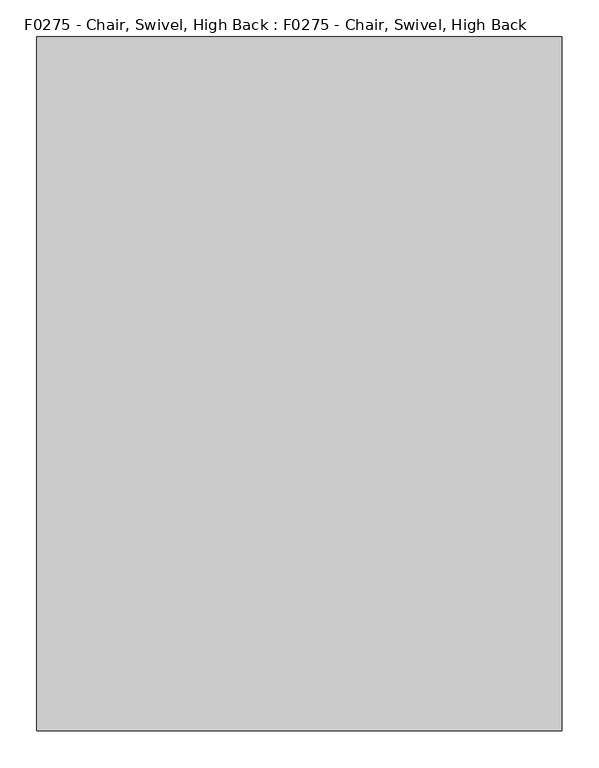
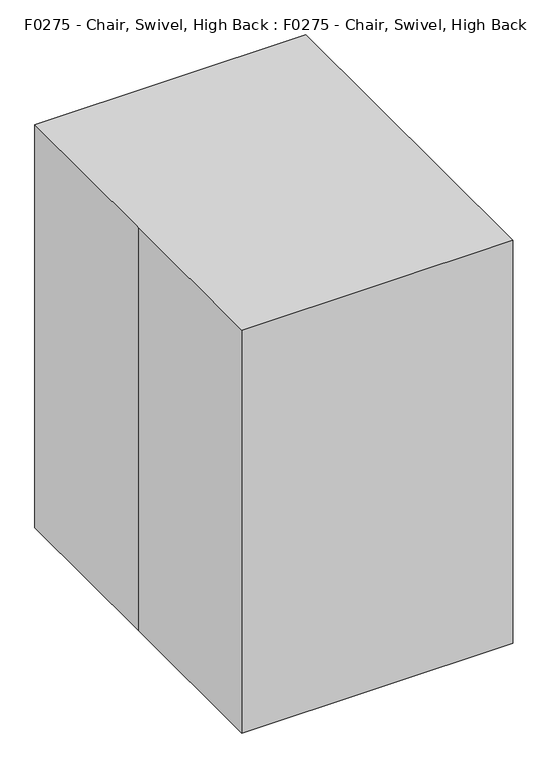
"""IFC4 building model written with IfcOpenShell, lengths in millimetres: proxy geometry, F0275 - Chair, Swivel, High Back : F0275 - Chair, Swivel, High Back."""

import ifcopenshell
import ifcopenshell.guid

model = None  # the IFC model being written
_history = None  # IfcOwnerHistory: only IFC2X3 demands one
_inside = {}  # id of a spatial element -> (the spatial element, [elements in it])
_under = {}  # id of a project, library or spatial element -> (it, [spatial elements below it])
_declared = {}  # id of a project -> (the project, [libraries it declares])
_typed = {}  # id of a type object -> (the type object, [elements of that type])
_made_of = {}  # id of a material, layer set ... -> (it, [elements and type objects made of it])


def new_model(schema):
    """Start an empty IFC model of exactly this schema.

    Asked for "IFC4X3", IfcOpenShell would pick the latest addendum, in which some entities
    have other attributes; the version numbers below select the first issue.
    IFC2X3 requires an IfcOwnerHistory on every rooted entity: one is made here for all.
    """
    global model, _history
    if schema == "IFC4X3":
        model = ifcopenshell.file(schema_version=(4, 3, 0, 0))
    else:
        model = ifcopenshell.file(schema=schema)
    _inside.clear()
    _under.clear()
    _declared.clear()
    _typed.clear()
    _made_of.clear()
    _history = None
    if model.schema == "IFC2X3":
        org = make("IfcOrganization", Name="unknown")
        user = make(
            "IfcPersonAndOrganization",
            ThePerson=make("IfcPerson", FamilyName="unknown"),
            TheOrganization=org,
        )
        app = make(
            "IfcApplication",
            ApplicationDeveloper=org,
            Version="unknown",
            ApplicationFullName="unknown",
            ApplicationIdentifier="unknown",
        )
        _history = make(
            "IfcOwnerHistory",
            OwningUser=user,
            OwningApplication=app,
            ChangeAction="ADDED",
            CreationDate=0,
        )
    return model


def make(cls, **values):
    """One entity of the class cls with the attributes given. An attribute that is None is left unset."""
    return model.create_entity(
        cls, **{name: value for name, value in values.items() if value is not None}
    )


def rooted(cls, **values):
    """An entity with a GlobalId (a new one), such as an element, a storey or a relation."""
    return make(cls, GlobalId=ifcopenshell.guid.new(), OwnerHistory=_history, **values)


def si_unit(unit_type, name, prefix=None):
    """IfcSIUnit, for example si_unit("LENGTHUNIT", "METRE", prefix="MILLI")."""
    return make("IfcSIUnit", UnitType=unit_type, Prefix=prefix, Name=name)


def assignment(units):
    """IfcUnitAssignment: the units of a project."""
    return None if units is None else make("IfcUnitAssignment", Units=units)


def point(xyz):
    """IfcCartesianPoint."""
    return None if xyz is None else make("IfcCartesianPoint", Coordinates=xyz)


def direction(xyz):
    """IfcDirection."""
    return None if xyz is None else make("IfcDirection", DirectionRatios=xyz)


def frame(location, z_axis=None, x_axis=None):
    """IfcAxis2Placement3D, a coordinate frame: its origin and axes. An axis left out is left unset."""
    return make(
        "IfcAxis2Placement3D",
        Location=point(location),
        Axis=direction(z_axis),
        RefDirection=direction(x_axis),
    )


def frame_2d(location, x_axis=None):
    """IfcAxis2Placement2D, a coordinate frame in the plane: its origin and x axis."""
    return make(
        "IfcAxis2Placement2D", Location=point(location), RefDirection=direction(x_axis)
    )


def origin():
    """The frame at (0, 0, 0) with its axes left unset."""
    return frame((0.0, 0.0, 0.0))


def origin_with_axes():
    """The frame at (0, 0, 0) with the z axis (0, 0, 1) and the x axis (1, 0, 0) written out."""
    return frame((0.0, 0.0, 0.0), z_axis=(0.0, 0.0, 1.0), x_axis=(1.0, 0.0, 0.0))


def place(relative_to, where):
    """IfcLocalPlacement: puts the frame where relative to a parent placement (None: the world)."""
    return make(
        "IfcLocalPlacement", PlacementRelTo=relative_to, RelativePlacement=where
    )


def context(
    kind, dimensions, precision=None, world=None, true_north=None, identifier=None
):
    """IfcGeometricRepresentationContext, for example the 3D "Model" context."""
    return make(
        "IfcGeometricRepresentationContext",
        ContextIdentifier=identifier,
        ContextType=kind,
        CoordinateSpaceDimension=dimensions,
        Precision=precision,
        WorldCoordinateSystem=world,
        TrueNorth=true_north,
    )


def project(units=None, contexts=None):
    """IfcProject with its units and contexts."""
    return rooted(
        "IfcProject",
        Name="project",
        RepresentationContexts=contexts,
        UnitsInContext=assignment(units),
    )


def spatial(cls, under=None, at=None, **own):
    """A site, building, storey or space (cls), placed at a placement, below another one or the project."""
    s = rooted(cls, ObjectPlacement=at, **own)
    if under is not None:
        _under.setdefault(under.id(), (under, []))[1].append(s)
    return s


def polyline(points):
    """IfcPolyline through the points."""
    return make("IfcPolyline", Points=[point(p) for p in points])


def circle_curve(where, radius):
    """IfcCircle in the frame where."""
    return make("IfcCircle", Position=where, Radius=radius)


def ellipse_curve(where, semi_axis1, semi_axis2):
    """IfcEllipse in the frame where."""
    return make(
        "IfcEllipse", Position=where, SemiAxis1=semi_axis1, SemiAxis2=semi_axis2
    )


def trimmed(basis, trim1, trim2, sense, master):
    """IfcTrimmedCurve: the piece of a basis curve between two trims."""
    return make(
        "IfcTrimmedCurve",
        BasisCurve=basis,
        Trim1=trim1,
        Trim2=trim2,
        SenseAgreement=sense,
        MasterRepresentation=master,
    )


def segment(curve, same_sense, transition):
    """IfcCompositeCurveSegment."""
    return make(
        "IfcCompositeCurveSegment",
        Transition=transition,
        SameSense=same_sense,
        ParentCurve=curve,
    )


def composite_curve(segments, self_intersect=None):
    """IfcCompositeCurve: segments joined end to end."""
    return make("IfcCompositeCurve", Segments=segments, SelfIntersect=self_intersect)


def outline(outer, holes=None, kind="AREA"):
    """IfcArbitraryClosedProfileDef: a profile drawn as a closed curve; with holes, ...WithVoids."""
    if holes is None:
        return make("IfcArbitraryClosedProfileDef", ProfileType=kind, OuterCurve=outer)
    return make(
        "IfcArbitraryProfileDefWithVoids",
        ProfileType=kind,
        OuterCurve=outer,
        InnerCurves=holes,
    )


def extrude(swept, where, along, depth):
    """IfcExtrudedAreaSolid: the profile swept, set in the frame where, extruded along a direction by depth."""
    return make(
        "IfcExtrudedAreaSolid",
        SweptArea=swept,
        Position=where,
        ExtrudedDirection=direction(along),
        Depth=depth,
    )


def shape(context_of_items, identifier, shape_type, items):
    """IfcShapeRepresentation: the items that make up one representation, for example the "Body"."""
    return make(
        "IfcShapeRepresentation",
        ContextOfItems=context_of_items,
        RepresentationIdentifier=identifier,
        RepresentationType=shape_type,
        Items=items,
    )


def source(mapping_origin, context_of_items, identifier, shape_type, items):
    """IfcRepresentationMap: a shape defined once, which mapped items show again and again."""
    return make(
        "IfcRepresentationMap",
        MappingOrigin=mapping_origin,
        MappedRepresentation=shape(context_of_items, identifier, shape_type, items),
    )


def transform(
    local_origin,
    x_axis=None,
    y_axis=None,
    z_axis=None,
    scale=None,
    scale2=None,
    scale3=None,
    uniform=True,
):
    """IfcCartesianTransformationOperator3D, or its non-uniform kind. x_axis, y_axis, z_axis: its Axis1, 2, 3."""
    if uniform:
        return make(
            "IfcCartesianTransformationOperator3D",
            Axis1=direction(x_axis),
            Axis2=direction(y_axis),
            LocalOrigin=point(local_origin),
            Scale=scale,
            Axis3=direction(z_axis),
        )
    return make(
        "IfcCartesianTransformationOperator3DnonUniform",
        Axis1=direction(x_axis),
        Axis2=direction(y_axis),
        LocalOrigin=point(local_origin),
        Scale=scale,
        Axis3=direction(z_axis),
        Scale2=scale2,
        Scale3=scale3,
    )


def mapped(mapping_source, mapping_target):
    """IfcMappedItem: shows the shape of a source again, moved by a transform."""
    return make(
        "IfcMappedItem", MappingSource=mapping_source, MappingTarget=mapping_target
    )


def made_of(thing, what):
    """Note that an element or type object is made of a material, layer set ...; save() writes the relation."""
    if what is not None:
        _made_of.setdefault(what.id(), (what, []))[1].append(thing)
    return thing


def element(
    cls,
    number,
    at=None,
    inside=None,
    cuts=None,
    type_object=None,
    material=None,
    context=None,
    identifier="Body",
    shape_type=None,
    held_by="IfcProductDefinitionShape",
    body=None,
    shapes=None,
    **own,
):
    """One element of the class cls, such as IfcWall. Its Tag is "e" and its number.

    at: its placement. inside: the storey or other place that contains it. cuts: it is an
    opening in that element (IfcRelVoidsElement). A single representation is given by context,
    identifier, shape_type and body (its items); several are given by shapes. held_by: the class
    of the entity that holds the representations. save() writes the other relations.
    """
    e = rooted(cls, Tag="e%d" % number, ObjectPlacement=at, **own)
    if body is not None:
        shapes = [shape(context, identifier, shape_type, body)]
    if shapes is not None:
        e.Representation = make(held_by, Representations=shapes)
    if inside is not None:
        _inside.setdefault(inside.id(), (inside, []))[1].append(e)
    if cuts is not None:
        rooted(
            "IfcRelVoidsElement", RelatingBuildingElement=cuts, RelatedOpeningElement=e
        )
    if type_object is not None:
        _typed.setdefault(type_object.id(), (type_object, []))[1].append(e)
    return made_of(e, material)


def aggregate(whole, parts):
    """IfcRelAggregates: a whole, such as a stair, and the parts it consists of."""
    return rooted("IfcRelAggregates", RelatingObject=whole, RelatedObjects=parts)


def save(model, path):
    """Write the relations noted so far, then the file.

    IfcRelAggregates (storeys below a building ...), IfcRelContainedInSpatialStructure (elements
    in a storey), IfcRelDefinesByType, IfcRelAssociatesMaterial and IfcRelDeclares: one each for
    every whole, place, type object, material and project.
    """
    for whole, parts in _under.values():
        aggregate(whole, parts)
    for where, things in _inside.values():
        rooted(
            "IfcRelContainedInSpatialStructure",
            RelatedElements=things,
            RelatingStructure=where,
        )
    for kind, things in _typed.values():
        rooted("IfcRelDefinesByType", RelatedObjects=things, RelatingType=kind)
    for what, things in _made_of.values():
        rooted("IfcRelAssociatesMaterial", RelatedObjects=things, RelatingMaterial=what)
    for by, libraries in _declared.values():
        rooted("IfcRelDeclares", RelatingContext=by, RelatedDefinitions=libraries)
    model.write(path)


def plane_surface(at):
    """IfcPlane: the flat surface through the origin of the frame at, square to its z axis."""
    return make("IfcPlane", Position=at)


def cylinder_surface(at, radius):
    """IfcCylindricalSurface: all points at the distance radius from the z axis of the frame at."""
    return make("IfcCylindricalSurface", Position=at, Radius=radius)


def revolved_surface(curve, axis_point, axis_direction):
    """IfcSurfaceOfRevolution: the curve turned about the line through axis_point along axis_direction."""
    return make(
        "IfcSurfaceOfRevolution",
        SweptCurve=make("IfcArbitraryOpenProfileDef", ProfileType="CURVE", Curve=curve),
        AxisPosition=make("IfcAxis1Placement", Location=point(axis_point), Axis=direction(axis_direction)),
    )


def advanced_brep(points, edges, surfaces, faces):
    """IfcAdvancedBrep: a solid bounded by faces that lie on surfaces and meet in shared edges.

    An edge is (start, end): straight between two places in points (the first is 0);
    or (start, end, curve); or (start, end, curve, False) where it runs against its curve.
    A face is (place in surfaces, loops), or (place, loops, False) where it looks against
    its surface's normal. A loop lists edges by number (the first is 1), with a minus sign
    where the edge is run from its end to its start. The first loop is the outer one.
    """
    corners = [point(p) for p in points]
    vertices = [make("IfcVertexPoint", VertexGeometry=c) for c in corners]
    made = []
    for start, end, *more in edges:
        made.append(
            make(
                "IfcEdgeCurve",
                EdgeStart=vertices[start],
                EdgeEnd=vertices[end],
                EdgeGeometry=more[0] if more else make("IfcPolyline", Points=[corners[start], corners[end]]),
                SameSense=more[1] if len(more) > 1 else True,
            )
        )
    hull = []
    for where, loops, *sense in faces:
        bounds = []
        for j, loop in enumerate(loops):
            ring = [make("IfcOrientedEdge", EdgeElement=made[abs(k) - 1], Orientation=k > 0) for k in loop]
            bounds.append(
                make(
                    "IfcFaceOuterBound" if j == 0 else "IfcFaceBound",
                    Bound=make("IfcEdgeLoop", EdgeList=ring),
                    Orientation=True,
                )
            )
        hull.append(make("IfcAdvancedFace", Bounds=bounds, FaceSurface=surfaces[where], SameSense=sense[0] if sense else True))
    return make("IfcAdvancedBrep", Outer=make("IfcClosedShell", CfsFaces=hull))


def f0275_chair_swivel_high_back_f0275_chair_swivel_high_back_15ce1d9b(model_context):
    return source(origin(), model_context, "Body", "SolidModel", [
        advanced_brep(
        [(-229.266219, -191.1122284, 430.2387079), (232.2634404, -190.6780441, 430.1937403), (236.5928369, -215.5732273, 432.7720849), (-229.266219, -216.744063, 432.893346), (-229.266219, -284.0352008, 957.2310718), (-229.266219, -307.2133069, 945.9699241), (236.5928369, -306.154555, 946.4843217), (232.2634404, -283.6425808, 957.4218273)],
        [
            (0, 1, circle_curve(frame((0.2419957, 1130.6870318, 293.3425871), z_axis=(0.0, 0.10301698777209904, 0.9946795967699162), x_axis=(-1.0, 0.0, 0.0)), 1348.5428628)),
            (1, 2, circle_curve(frame((232.2634404, -203.4980924, 431.5214872), z_axis=(0.0, -0.10301698777209904, -0.9946795967699162), x_axis=(-1.0, 0.0, 0.0)), 12.888621)),
            (2, 3, circle_curve(frame((0.2419957, 1130.6870318, 293.3425871), z_axis=(0.0, -0.10301698777209904, -0.9946795967699162), x_axis=(-1.0, 0.0, 0.0)), 1373.9428628)),
            (3, 0, circle_curve(frame((-229.266219, -203.9281457, 431.5660269), z_axis=(0.0, -0.10301698777209904, -0.9946795967699162), x_axis=(-1.0, 0.0, 0.0)), 12.8844679)),
            (4, 5, circle_curve(frame((-229.266219, -295.6242538, 951.6004979), z_axis=(0.0, -0.4370047614753819, 0.8994591922082094), x_axis=(-1.0, 0.0, 0.0)), 12.8844679)),
            (5, 6, circle_curve(frame((0.2419957, 911.2285794, 1537.9533187), z_axis=(0.0, -0.4370047614753819, 0.8994591922082094), x_axis=(-1.0, 0.0, 0.0)), 1373.9428628)),
            (6, 7, circle_curve(frame((232.2634404, -295.2353694, 951.7894385), z_axis=(0.0, -0.4370047614753819, 0.8994591922082094), x_axis=(-1.0, 0.0, 0.0)), 12.888621)),
            (7, 4, circle_curve(frame((0.2419957, 911.2285794, 1537.9533187), z_axis=(0.0, 0.4370047614753819, -0.8994591922082094), x_axis=(-1.0, 0.0, 0.0)), 1348.5428628)),
            (7, 1, circle_curve(frame((232.2634404, -1161.7926736, 530.7701512), z_axis=(-1.0, 0.0, 0.0), x_axis=(0.0, 0.9946795967699159, -0.10301698777210248)), 976.308987)),
            (0, 4, circle_curve(frame((-229.266219, -1161.7926736, 530.7701512), z_axis=(1.0, 0.0, 0.0), x_axis=(0.0, 0.9946795967699159, -0.10301698777210248)), 975.8724803)),
            (6, 2, circle_curve(frame((236.5928369, -1161.7926736, 530.7701512), z_axis=(-1.0, 0.0, 0.0), x_axis=(0.0, 0.9946795967699159, -0.10301698777210248)), 951.280643)),
            (5, 3, circle_curve(frame((-229.266219, -1161.7926736, 530.7701512), z_axis=(-1.0, 0.0, 0.0), x_axis=(0.0, 0.9946795967699159, -0.10301698777210248)), 950.1035446)),
        ],
        [
            plane_surface(frame((-317.2580043, -172.9739127, 428.3601586), z_axis=(0.0, -0.10301698777210244, -0.9946795967699159), x_axis=(-1.0, 0.0, 0.0))),
            plane_surface(frame((-317.2580043, -267.633261, 965.2), z_axis=(0.0, -0.437004761475379, 0.8994591922082108), x_axis=(-1.0, 0.0, 0.0))),
            revolved_surface(trimmed(ellipse_curve(frame((0.2419957, 1130.6870318, 293.3425871), z_axis=(0.0, 0.10301698777209904, 0.9946795967699162), x_axis=(-1.0, 0.0, 0.0)), 1348.5428628, 1348.5428628), [point((-229.266219, -191.1122284, 430.2387079))], [point((232.2634404, -190.6780441, 430.1937403))], True, "CARTESIAN"), (-317.2580043, -1161.7926736, 530.7701512), (1.0, 0.0, 0.0)),
            revolved_surface(trimmed(ellipse_curve(frame((232.2634404, -203.4980924, 431.5214872), z_axis=(0.0, -0.10301698777209904, -0.9946795967699162), x_axis=(-1.0, 0.0, 0.0)), 12.888621, 12.888621), [point((232.2634404, -190.6780441, 430.1937403))], [point((236.5928369, -215.5732273, 432.7720849))], True, "CARTESIAN"), (-317.2580043, -1161.7926736, 530.7701512), (1.0, 0.0, 0.0)),
            revolved_surface(trimmed(ellipse_curve(frame((0.2419957, 1130.6870318, 293.3425871), z_axis=(0.0, -0.10301698777209904, -0.9946795967699162), x_axis=(-1.0, 0.0, 0.0)), 1373.9428628, 1373.9428628), [point((236.5928369, -215.5732273, 432.7720849))], [point((-229.266219, -216.744063, 432.893346))], True, "CARTESIAN"), (-317.2580043, -1161.7926736, 530.7701512), (1.0, 0.0, 0.0)),
            revolved_surface(trimmed(ellipse_curve(frame((-229.266219, -203.9281457, 431.5660269), z_axis=(0.0, -0.10301698777209904, -0.9946795967699162), x_axis=(-1.0, 0.0, 0.0)), 12.8844679, 12.8844679), [point((-229.266219, -216.744063, 432.893346))], [point((-229.266219, -191.1122284, 430.2387079))], True, "CARTESIAN"), (-317.2580043, -1161.7926736, 530.7701512), (1.0, 0.0, 0.0)),
        ],
        [
            (0, [[1, 2, 3, 4]]),
            (1, [[5, 6, 7, 8]]),
            (2, [[9, -1, 10, -8]]),
            (3, [[11, -2, -9, -7]]),
            (4, [[12, -3, -11, -6]]),
            (5, [[-10, -4, -12, -5]]),
        ],
    ),
        extrude(outline(composite_curve([segment(polyline([(-212.8377573, -173.8554076), (-212.8377573, 183.0901052)]), True, "CONTINUOUS"), segment(trimmed(circle_curve(frame_2d((-186.0922445, 183.0901052)), 26.7455128), [point((-212.8377573, 183.0901052))], [point((-186.0922445, 209.835618))], False, "CARTESIAN"), True, "CONTINUOUS"), segment(polyline([(-186.0922445, 209.835618), (194.9077555, 209.835618)]), True, "CONTINUOUS"), segment(trimmed(circle_curve(frame_2d((194.9077555, 183.0901052)), 26.7455128), [point((194.9077555, 209.835618))], [point((221.6532683, 183.0901052))], False, "CARTESIAN"), True, "CONTINUOUS"), segment(polyline([(221.6532683, 183.0901052), (221.6532683, -173.8554076), (-212.8377573, -173.8554076)]), True, "CONTINUOUS")], self_intersect=False)), frame((0.0, 0.0, 324.0440254), z_axis=(0.0, 0.0, 1.0), x_axis=(1.0, 0.0, 0.0)), (0.0, 0.0, 1.0), 67.8491407),
        advanced_brep(
        [(-212.8377573, -172.5098948, 391.8931661), (-211.4922445, -173.8554076, 391.8931661), (-211.4922445, -173.8554076, 324.0440254), (-212.8377573, -172.5098948, 324.0440254), (-212.8377573, 183.0901052, 324.0440254), (-212.8377573, 183.0901052, 391.8931661), (-186.0922445, 209.835618, 391.8931661), (-186.0922445, 209.835618, 324.0440254), (194.9077555, 209.835618, 324.0440254), (194.9077555, 209.835618, 391.8931661), (221.6532683, 183.0901052, 391.8931661), (221.6532683, 183.0901052, 324.0440254), (221.6532683, -172.5098948, 324.0440254), (221.6532683, -172.5098948, 391.8931661), (220.3077555, -173.8554076, 391.8931661), (220.3077555, -173.8554076, 324.0440254)],
        [
            (0, 1, circle_curve(frame((-211.4922445, -172.5098948, 391.8931661), z_axis=(0.0, 0.0, 1.0), x_axis=(0.0, -1.0, 0.0)), 1.3455128)),
            (1, 2),
            (2, 3, circle_curve(frame((-211.4922445, -172.5098948, 324.0440254), z_axis=(0.0, 0.0, -1.0), x_axis=(0.0, -1.0, 0.0)), 1.3455128)),
            (3, 0),
            (2, 1, circle_curve(frame((-211.4922445, -173.8554076, 357.9685958), z_axis=(-1.0, 0.0, 0.0), x_axis=(0.0, 1.0, 0.0)), 33.9245703)),
            (0, 3, circle_curve(frame((-212.8377573, -172.5098948, 357.9685958), z_axis=(0.0, -1.0, 0.0), x_axis=(1.0, 0.0, 0.0)), 33.9245703)),
            (3, 4),
            (4, 5),
            (5, 0),
            (5, 4, circle_curve(frame((-212.8377573, 183.0901052, 357.9685958), z_axis=(0.0, -1.0, 0.0), x_axis=(1.0, 0.0, 0.0)), 33.9245703)),
            (6, 5, circle_curve(frame((-186.0922445, 183.0901052, 391.8931661), z_axis=(0.0, 0.0, 1.0), x_axis=(-1.0, 0.0, 0.0)), 26.7455128)),
            (4, 7, circle_curve(frame((-186.0922445, 183.0901052, 324.0440254), z_axis=(0.0, 0.0, -1.0), x_axis=(-1.0, 0.0, 0.0)), 26.7455128)),
            (7, 6),
            (6, 7, circle_curve(frame((-186.0922445, 209.835618, 357.9685958), z_axis=(-1.0, 0.0, 0.0), x_axis=(0.0, -1.0, 0.0)), 33.9245703)),
            (7, 8),
            (8, 9),
            (9, 6),
            (9, 8, circle_curve(frame((194.9077555, 209.835618, 357.9685958), z_axis=(-1.0, 0.0, 0.0), x_axis=(0.0, -1.0, 0.0)), 33.9245703)),
            (10, 9, circle_curve(frame((194.9077555, 183.0901052, 391.8931661), z_axis=(0.0, 0.0, 1.0), x_axis=(0.0, 1.0, 0.0)), 26.7455128)),
            (8, 11, circle_curve(frame((194.9077555, 183.0901052, 324.0440254), z_axis=(0.0, 0.0, -1.0), x_axis=(0.0, 1.0, 0.0)), 26.7455128)),
            (11, 10),
            (10, 11, circle_curve(frame((221.6532683, 183.0901052, 357.9685958), z_axis=(0.0, 1.0, 0.0), x_axis=(-1.0, 0.0, 0.0)), 33.9245703)),
            (11, 12),
            (12, 13),
            (13, 10),
            (13, 12, circle_curve(frame((221.6532683, -172.5098948, 357.9685958), z_axis=(0.0, 1.0, 0.0), x_axis=(-1.0, 0.0, 0.0)), 33.9245703)),
            (14, 13, circle_curve(frame((220.3077555, -172.5098948, 391.8931661), z_axis=(0.0, 0.0, 1.0), x_axis=(1.0, 0.0, 0.0)), 1.3455128)),
            (12, 15, circle_curve(frame((220.3077555, -172.5098948, 324.0440254), z_axis=(0.0, 0.0, -1.0), x_axis=(1.0, 0.0, 0.0)), 1.3455128)),
            (15, 14),
            (14, 15, circle_curve(frame((220.3077555, -173.8554076, 357.9685958), z_axis=(1.0, 0.0, 0.0), x_axis=(0.0, 1.0, 0.0)), 33.9245703)),
            (15, 2),
            (1, 14),
        ],
        [
            revolved_surface(polyline([(-211.4922445, -173.8554076, 324.0440254), (-211.4922445, -173.8554076, 391.8931661)]), (-211.4922445, -172.5098948, 0.0), (0.0, 0.0, -1.0)),
            revolved_surface(trimmed(ellipse_curve(frame((-211.4922445, -173.8554076, 357.9685958), z_axis=(1.0, 0.0, 0.0), x_axis=(0.0, 1.0, 0.0)), 33.9245703, 33.9245703), [point((-211.4922445, -173.8554076, 391.8931661))], [point((-211.4922445, -173.8554076, 324.0440254))], True, "CARTESIAN"), (-211.4922445, -172.5098948, 0.0), (0.0, 0.0, -1.0)),
            plane_surface(frame((-212.8377573, -172.5098948, 324.0440254), z_axis=(1.0, 0.0, 0.0), x_axis=(0.0, 1.0, 0.0))),
            cylinder_surface(frame((-212.8377573, -172.5098948, 357.9685958), z_axis=(0.0, -1.0, 0.0), x_axis=(1.0, 0.0, 0.0)), 33.9245703),
            revolved_surface(polyline([(-212.8377573, 183.0901052, 324.0440254), (-212.8377573, 183.0901052, 391.8931661)]), (-186.0922445, 183.0901052, 0.0), (0.0, 0.0, -1.0)),
            revolved_surface(trimmed(ellipse_curve(frame((-212.8377573, 183.0901052, 357.9685958), z_axis=(0.0, -1.0, 0.0), x_axis=(1.0, 0.0, 0.0)), 33.9245703, 33.9245703), [point((-212.8377573, 183.0901052, 391.8931661))], [point((-212.8377573, 183.0901052, 324.0440254))], True, "CARTESIAN"), (-186.0922445, 183.0901052, 0.0), (0.0, 0.0, -1.0)),
            plane_surface(frame((-186.0922445, 209.835618, 324.0440254), z_axis=(0.0, -1.0, 0.0), x_axis=(1.0, 0.0, 0.0))),
            cylinder_surface(frame((-186.0922445, 209.835618, 357.9685958), z_axis=(-1.0, 0.0, 0.0), x_axis=(0.0, -1.0, 0.0)), 33.9245703),
            revolved_surface(polyline([(194.9077555, 209.835618, 324.0440254), (194.9077555, 209.835618, 391.8931661)]), (194.9077555, 183.0901052, 0.0), (0.0, 0.0, -1.0)),
            revolved_surface(trimmed(ellipse_curve(frame((194.9077555, 209.835618, 357.9685958), z_axis=(-1.0, 0.0, 0.0), x_axis=(0.0, -1.0, 0.0)), 33.9245703, 33.9245703), [point((194.9077555, 209.835618, 391.8931661))], [point((194.9077555, 209.835618, 324.0440254))], True, "CARTESIAN"), (194.9077555, 183.0901052, 0.0), (0.0, 0.0, -1.0)),
            plane_surface(frame((221.6532683, 183.0901052, 324.0440254), z_axis=(-1.0, 0.0, 0.0), x_axis=(0.0, -1.0, 0.0))),
            cylinder_surface(frame((221.6532683, 183.0901052, 357.9685958), z_axis=(0.0, 1.0, 0.0), x_axis=(-1.0, 0.0, 0.0)), 33.9245703),
            revolved_surface(polyline([(221.6532683, -172.5098948, 324.0440254), (221.6532683, -172.5098948, 391.8931661)]), (220.3077555, -172.5098948, 0.0), (0.0, 0.0, -1.0)),
            revolved_surface(trimmed(ellipse_curve(frame((221.6532683, -172.5098948, 357.9685958), z_axis=(0.0, 1.0, 0.0), x_axis=(-1.0, 0.0, 0.0)), 33.9245703, 33.9245703), [point((221.6532683, -172.5098948, 391.8931661))], [point((221.6532683, -172.5098948, 324.0440254))], True, "CARTESIAN"), (220.3077555, -172.5098948, 0.0), (0.0, 0.0, -1.0)),
            plane_surface(frame((220.3077555, -173.8554076, 324.0440254), z_axis=(0.0, 1.0, 0.0), x_axis=(-1.0, 0.0, 0.0))),
            cylinder_surface(frame((220.3077555, -173.8554076, 357.9685958), z_axis=(1.0, 0.0, 0.0), x_axis=(0.0, 1.0, 0.0)), 33.9245703),
        ],
        [
            (0, [[1, 2, 3, 4]]),
            (1, [[-3, 5, -1, 6]]),
            (2, [[-4, 7, 8, 9]]),
            (3, [[-6, -9, 10, -7]]),
            (4, [[11, -8, 12, 13]]),
            (5, [[-12, -10, -11, 14]]),
            (6, [[-13, 15, 16, 17]]),
            (7, [[-14, -17, 18, -15]]),
            (8, [[19, -16, 20, 21]]),
            (9, [[-20, -18, -19, 22]]),
            (10, [[-21, 23, 24, 25]]),
            (11, [[-22, -25, 26, -23]]),
            (12, [[27, -24, 28, 29]]),
            (13, [[-28, -26, -27, 30]]),
            (14, [[-29, 31, -2, 32]]),
            (15, [[-30, -32, -5, -31]]),
        ],
    ),
        extrude(outline(composite_curve([segment(trimmed(circle_curve(frame_2d((0.2419957, 0.182522)), 12.7), [point((12.9419957, 0.182522))], [point((-12.4580043, 0.182522))], False, "CARTESIAN"), True, "CONTINUOUS"), segment(trimmed(circle_curve(frame_2d((0.2419957, 0.182522)), 12.7), [point((-12.4580043, 0.182522))], [point((12.9419957, 0.182522))], False, "CARTESIAN"), True, "CONTINUOUS")], self_intersect=False)), frame((0.0, 0.0, 212.7487443), z_axis=(0.0, 0.0, 1.0), x_axis=(1.0, 0.0, 0.0)), (0.0, 0.0, 1.0), 66.217703),
        extrude(outline(polyline([(-355.6, 469.9), (355.6, 469.9), (355.6, -469.9), (-355.6, -469.9), (-355.6, 0.0), (-355.6, 469.9)])), origin_with_axes(), (0.0, 0.0, 1.0), 1117.6),
    ])


if __name__ == "__main__":
    model = new_model("IFC4")
    model_context = context("Model", 3, world=origin())
    ifc_project = project(units=[si_unit("LENGTHUNIT", "METRE", prefix="MILLI")], contexts=[model_context])
    site = spatial("IfcSite", under=ifc_project)
    building = spatial("IfcBuilding", under=site)
    placement = place(None, origin())
    f0275_chair_swivel_high_back_f0275_chair_swivel_high_back_shape = f0275_chair_swivel_high_back_f0275_chair_swivel_high_back_15ce1d9b(model_context)
    element("IfcBuildingElementProxy", 1, Name="F0275 - Chair, Swivel, High Back : F0275 - Chair, Swivel, High Back", ObjectType="F0275 - Chair, Swivel, High Back : F0275 - Chair, Swivel, High Back", at=placement, inside=building, context=model_context, shape_type="MappedRepresentation", body=[
        mapped(f0275_chair_swivel_high_back_f0275_chair_swivel_high_back_shape, transform((0.0, 0.0, 0.0), x_axis=(1.0, 0.0, 0.0), y_axis=(0.0, 1.0, 0.0), z_axis=(0.0, 0.0, 1.0))),
    ])
    save(model, "model.ifc")

# Revit data of these elements
# Project information
#   Sheets - Total = "5"
#   Project Issue Date = "Issue Date"
#   Project Status = "Project Status"
#   Client Name = "Owner"
#   Project Address = "Enter address here"
#   Project Name = "Project Name"
#   Project Number = "Project Number"
#   Publication Date = "30-Jan-15"
# Type "F0275 - Chair, Swivel, High Back : F0275 - Chair, Swivel, High Back"
#   Watts2 = "0"
#   Watts1 = "0"
#   Unit_Issue = "EA"
#   UTIL_6_Misc = "-"
#   UTIL_5_NonMedGas = "-"
#   UTIL_4_MiscGas = "-"
#   UTIL_3_MedGas = "-"
#   UTIL_2_Elec = "-"
#   UTIL_1_WaterDrain = "-"
#   Nomenclature = "Chair, Swivel, High Back"
#   NSN = "7110"
#   Location [instance default] = ""
#   JSN = "F0275"
#   Fund_Source_VA = "-"
#   Fund_Source_Navy = "-"
#   Fund_Source_Army = "-"
#   Fund_Source_AF = "-"
#   ELEC_Volts2 = "0"
#   ELEC_Volts1 = "0"
#   ELEC_Phase2 = "0"
#   ELEC_Phase1 = "0"
#   ELEC_HertzSwitch = "0"
#   ELEC_HertzDependent = "0"
#   ELEC_Hertz = "0"
#   ELEC_Amps2 = "0"
#   ELEC_Amps1 = "0"
#   DetailDescription = "Highback contemporary swivel chair, 41\" high X 23\" wide X 23\" deep with five (5) caster swivel base and arms. Chair may be used at desks or in conference rooms. Back and seat are foam padded and upholstered with either woven textile fabric or vinyl."
#   CAT_VA = "C"
#   CAT_Navy = "C"
#   CAT_IHS = "-"
#   CAT_Army = "C"
#   CAT_AF = "C"
#   BTUperhour = "0"
#   Weight_IP = 56
#   DIM_Width_IP = 2' - 4"
#   DIM_Height_IP = 3' - 8"
#   DIM_Depth_IP = 3' - 1"
# Element 1 (IfcBuildingElementProxy, "F0275 - Chair, Swivel, High Back : F0275 - Chair, Swivel, High Back")
#   Location = "OFD01"
#   Materials on its faces: "00 - bernhardt blitz - base", "00 - bernhardt blitz - Seat Fabric", "00 - bernhardt blitz - wheels", "00 - bernhardt blitz - arms", "00 - bernhardt blitz - mechanic", "EquipSpace", "00 - bernhardt blitz - Back Fabric"
# Materials
#   "00 - bernhardt blitz - base": class "Miscellaneous", colour RGB 192 192 192, transparency 0
#   "00 - bernhardt blitz - Seat Fabric": class "Miscellaneous", colour RGB 188 173 117, transparency 0
#   "00 - bernhardt blitz - wheels": class "Miscellaneous", colour RGB 51 51 51, transparency 0
#   "00 - bernhardt blitz - arms": class "Miscellaneous", colour RGB 51 51 51, transparency 0
#   "00 - bernhardt blitz - mechanic": class "Miscellaneous", colour RGB 62 62 62, transparency 0
#   "EquipSpace": class "Unassigned", colour RGB 221 217 195, transparency 0.5
#   "00 - bernhardt blitz - Back Fabric": class "Miscellaneous", colour RGB 93 93 93, transparency 0
